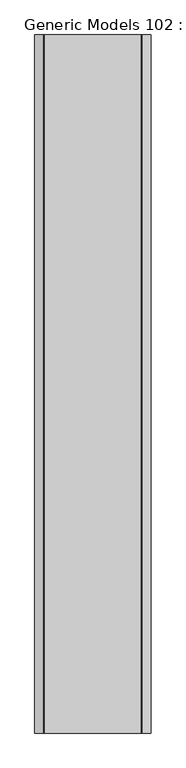
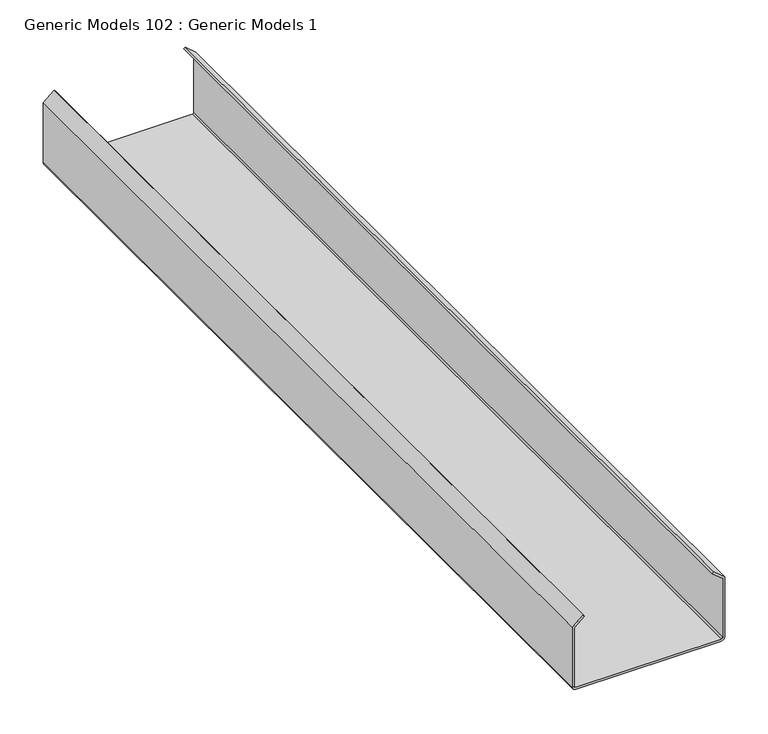
"""IFC4 building model written with IfcOpenShell, lengths in millimetres: proxy geometry, Generic Models 102 : Generic Models 1."""

from ifc_helpers import new_model, si_unit, point, frame, frame_2d, origin, place, context, project, spatial, polyline, circle_curve, trimmed, segment, composite_curve, outline, extrude, source, transform, mapped, element, save


def generic_models_102_generic_models_1_dd9ddf13(model_context):
    return source(origin(), model_context, "Body", "SweptSolid", [
        extrude(outline(composite_curve([segment(polyline([(2574.1308044, 55088.8446108), (2586.3759084, 55074.2514642), (2584.2477412, 55072.4657198), (2572.8353435, 55086.0664858), (2489.9204476, 55086.0664858)]), True, "CONTINUOUS"), segment(trimmed(circle_curve(frame_2d((2489.9939735, 55084.0828039)), 1.9850441), [point((2489.9204476, 55086.0664858))], [point((2488.0089294, 55084.0828039))], True, "CARTESIAN"), True, "CONTINUOUS"), segment(polyline([(2488.0089294, 55084.0828039), (2488.0089294, 54890.4056769)]), True, "CONTINUOUS"), segment(trimmed(circle_curve(frame_2d((2489.9946693, 54890.4056769)), 1.9857399), [point((2488.0089294, 54890.4056769))], [point((2489.8892776, 54888.4227358))], True, "CARTESIAN"), True, "CONTINUOUS"), segment(polyline([(2489.8892776, 54888.4227358), (2572.8353435, 54888.4227358), (2584.2709644, 54902.0511782), (2586.3991316, 54900.2654338), (2574.1308044, 54885.6446108), (2489.9933044, 54885.6446108)]), True, "CONTINUOUS"), segment(trimmed(circle_curve(frame_2d((2489.9933044, 54890.4071108)), 4.7625), [point((2489.9933044, 54885.6446108))], [point((2485.2308044, 54890.4071108))], False, "CARTESIAN"), True, "CONTINUOUS"), segment(polyline([(2485.2308044, 54890.4071108), (2485.2308044, 55084.0821108)]), True, "CONTINUOUS"), segment(trimmed(circle_curve(frame_2d((2489.9933044, 55084.0821108)), 4.7625), [point((2485.2308044, 55084.0821108))], [point((2489.9933044, 55088.8446108))], False, "CARTESIAN"), True, "CONTINUOUS"), segment(polyline([(2489.9933044, 55088.8446108), (2574.1308044, 55088.8446108)]), True, "CONTINUOUS")], self_intersect=False)), frame((0.0, 0.0, 0.0), z_axis=(0.0, 1.0, 0.0), x_axis=(0.0, 0.0, 1.0)), (0.0, 0.0, 1.0), 1219.2),
    ])


if __name__ == "__main__":
    model = new_model("IFC4")
    model_context = context("Model", 3, world=origin())
    ifc_project = project(units=[si_unit("LENGTHUNIT", "METRE", prefix="MILLI")], contexts=[model_context])
    site = spatial("IfcSite", under=ifc_project)
    building = spatial("IfcBuilding", under=site)
    placement = place(None, origin())
    generic_models_102_generic_models_1_shape = generic_models_102_generic_models_1_dd9ddf13(model_context)
    element("IfcBuildingElementProxy", 1, Name="Generic Models 102 : Generic Models 1", ObjectType="Generic Models 102 : Generic Models 1", at=placement, inside=building, context=model_context, shape_type="MappedRepresentation", body=[
        mapped(generic_models_102_generic_models_1_shape, transform((0.0, 0.0, 0.0), x_axis=(1.0, 0.0, 0.0), y_axis=(0.0, 1.0, 0.0), z_axis=(0.0, 0.0, 1.0))),
    ])
    save(model, "model.ifc")

# Revit data of these elements
# Element 1 (IfcBuildingElementProxy, "Generic Models 102 : Generic Models 1")
#   Materials on its faces: "EXISTING GIRT"
# Materials
#   "EXISTING GIRT": class "Metal", colour RGB 199 199 199, transparency 0, Description = "Carbon steel", Cost = 0
